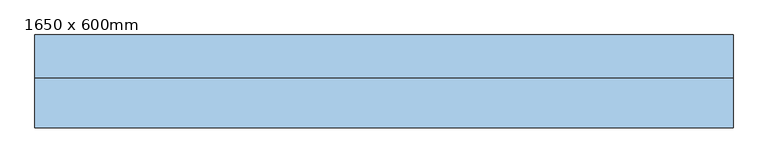
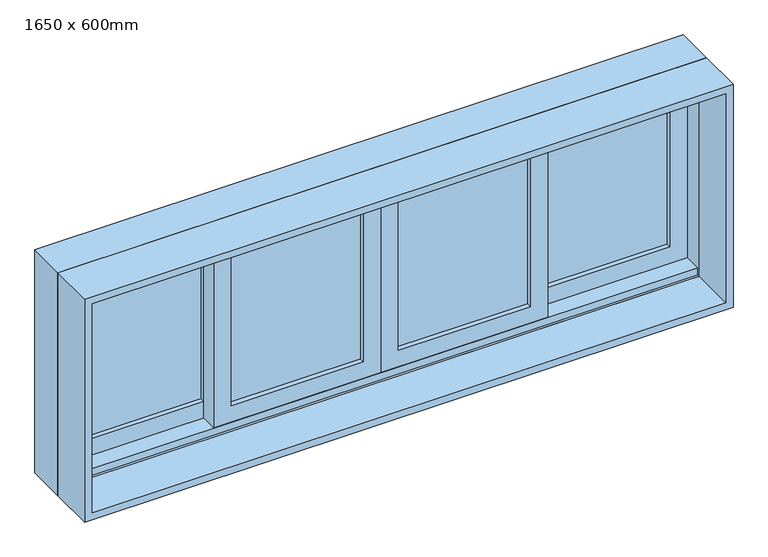
"""IFC4 building model written with IfcOpenShell, lengths in millimetres: window geometry, Janela-deslizante-quatro : 1650 x 600mm."""

import ifcopenshell
import ifcopenshell.guid

model = None  # the IFC model being written
_history = None  # IfcOwnerHistory: only IFC2X3 demands one
_inside = {}  # id of a spatial element -> (the spatial element, [elements in it])
_under = {}  # id of a project, library or spatial element -> (it, [spatial elements below it])
_declared = {}  # id of a project -> (the project, [libraries it declares])
_typed = {}  # id of a type object -> (the type object, [elements of that type])
_made_of = {}  # id of a material, layer set ... -> (it, [elements and type objects made of it])


def new_model(schema):
    """Start an empty IFC model of exactly this schema.

    Asked for "IFC4X3", IfcOpenShell would pick the latest addendum, in which some entities
    have other attributes; the version numbers below select the first issue.
    IFC2X3 requires an IfcOwnerHistory on every rooted entity: one is made here for all.
    """
    global model, _history
    if schema == "IFC4X3":
        model = ifcopenshell.file(schema_version=(4, 3, 0, 0))
    else:
        model = ifcopenshell.file(schema=schema)
    _inside.clear()
    _under.clear()
    _declared.clear()
    _typed.clear()
    _made_of.clear()
    _history = None
    if model.schema == "IFC2X3":
        org = make("IfcOrganization", Name="unknown")
        user = make(
            "IfcPersonAndOrganization",
            ThePerson=make("IfcPerson", FamilyName="unknown"),
            TheOrganization=org,
        )
        app = make(
            "IfcApplication",
            ApplicationDeveloper=org,
            Version="unknown",
            ApplicationFullName="unknown",
            ApplicationIdentifier="unknown",
        )
        _history = make(
            "IfcOwnerHistory",
            OwningUser=user,
            OwningApplication=app,
            ChangeAction="ADDED",
            CreationDate=0,
        )
    return model


def make(cls, **values):
    """One entity of the class cls with the attributes given. An attribute that is None is left unset."""
    return model.create_entity(
        cls, **{name: value for name, value in values.items() if value is not None}
    )


def rooted(cls, **values):
    """An entity with a GlobalId (a new one), such as an element, a storey or a relation."""
    return make(cls, GlobalId=ifcopenshell.guid.new(), OwnerHistory=_history, **values)


def si_unit(unit_type, name, prefix=None):
    """IfcSIUnit, for example si_unit("LENGTHUNIT", "METRE", prefix="MILLI")."""
    return make("IfcSIUnit", UnitType=unit_type, Prefix=prefix, Name=name)


def assignment(units):
    """IfcUnitAssignment: the units of a project."""
    return None if units is None else make("IfcUnitAssignment", Units=units)


def point(xyz):
    """IfcCartesianPoint."""
    return None if xyz is None else make("IfcCartesianPoint", Coordinates=xyz)


def direction(xyz):
    """IfcDirection."""
    return None if xyz is None else make("IfcDirection", DirectionRatios=xyz)


def frame(location, z_axis=None, x_axis=None):
    """IfcAxis2Placement3D, a coordinate frame: its origin and axes. An axis left out is left unset."""
    return make(
        "IfcAxis2Placement3D",
        Location=point(location),
        Axis=direction(z_axis),
        RefDirection=direction(x_axis),
    )


def origin():
    """The frame at (0, 0, 0) with its axes left unset."""
    return frame((0.0, 0.0, 0.0))


def place(relative_to, where):
    """IfcLocalPlacement: puts the frame where relative to a parent placement (None: the world)."""
    return make(
        "IfcLocalPlacement", PlacementRelTo=relative_to, RelativePlacement=where
    )


def context(
    kind, dimensions, precision=None, world=None, true_north=None, identifier=None
):
    """IfcGeometricRepresentationContext, for example the 3D "Model" context."""
    return make(
        "IfcGeometricRepresentationContext",
        ContextIdentifier=identifier,
        ContextType=kind,
        CoordinateSpaceDimension=dimensions,
        Precision=precision,
        WorldCoordinateSystem=world,
        TrueNorth=true_north,
    )


def project(units=None, contexts=None):
    """IfcProject with its units and contexts."""
    return rooted(
        "IfcProject",
        Name="project",
        RepresentationContexts=contexts,
        UnitsInContext=assignment(units),
    )


def spatial(cls, under=None, at=None, **own):
    """A site, building, storey or space (cls), placed at a placement, below another one or the project."""
    s = rooted(cls, ObjectPlacement=at, **own)
    if under is not None:
        _under.setdefault(under.id(), (under, []))[1].append(s)
    return s


def polyline(points):
    """IfcPolyline through the points."""
    return make("IfcPolyline", Points=[point(p) for p in points])


def outline(outer, holes=None, kind="AREA"):
    """IfcArbitraryClosedProfileDef: a profile drawn as a closed curve; with holes, ...WithVoids."""
    if holes is None:
        return make("IfcArbitraryClosedProfileDef", ProfileType=kind, OuterCurve=outer)
    return make(
        "IfcArbitraryProfileDefWithVoids",
        ProfileType=kind,
        OuterCurve=outer,
        InnerCurves=holes,
    )


def extrude(swept, where, along, depth):
    """IfcExtrudedAreaSolid: the profile swept, set in the frame where, extruded along a direction by depth."""
    return make(
        "IfcExtrudedAreaSolid",
        SweptArea=swept,
        Position=where,
        ExtrudedDirection=direction(along),
        Depth=depth,
    )


def faces_of(points, faces, orient=None, outer=None):
    """IfcFace entities. A face is a list of loops; a loop is a list of indices into points, from 0.

    orient and outer hold one flag for each loop. By default every Orientation is true, the
    first loop of a face is its IfcFaceOuterBound and the others are IfcFaceBound.
    """
    made = []
    for i, loops in enumerate(faces):
        bounds = []
        for j, loop in enumerate(loops):
            is_outer = j == 0 if outer is None else outer[i][j]
            bounds.append(
                make(
                    "IfcFaceOuterBound" if is_outer else "IfcFaceBound",
                    Bound=make("IfcPolyLoop", Polygon=[points[k] for k in loop]),
                    Orientation=True if orient is None else orient[i][j],
                )
            )
        made.append(make("IfcFace", Bounds=bounds))
    return made


def faceted_brep(points, faces, orient=None, outer=None, voids=None):
    """IfcFacetedBrep: a solid bounded by flat faces; with voids (closed shells), ...WithVoids."""
    shared = [point(p) for p in points]
    hull = make("IfcClosedShell", CfsFaces=faces_of(shared, faces, orient, outer))
    if voids is None:
        return make("IfcFacetedBrep", Outer=hull)
    return make(
        "IfcFacetedBrepWithVoids",
        Outer=hull,
        Voids=[
            make(cls, CfsFaces=faces_of(shared, fs, o, b)) for cls, fs, o, b in voids
        ],
    )


def shape(context_of_items, identifier, shape_type, items):
    """IfcShapeRepresentation: the items that make up one representation, for example the "Body"."""
    return make(
        "IfcShapeRepresentation",
        ContextOfItems=context_of_items,
        RepresentationIdentifier=identifier,
        RepresentationType=shape_type,
        Items=items,
    )


def source(mapping_origin, context_of_items, identifier, shape_type, items):
    """IfcRepresentationMap: a shape defined once, which mapped items show again and again."""
    return make(
        "IfcRepresentationMap",
        MappingOrigin=mapping_origin,
        MappedRepresentation=shape(context_of_items, identifier, shape_type, items),
    )


def transform(
    local_origin,
    x_axis=None,
    y_axis=None,
    z_axis=None,
    scale=None,
    scale2=None,
    scale3=None,
    uniform=True,
):
    """IfcCartesianTransformationOperator3D, or its non-uniform kind. x_axis, y_axis, z_axis: its Axis1, 2, 3."""
    if uniform:
        return make(
            "IfcCartesianTransformationOperator3D",
            Axis1=direction(x_axis),
            Axis2=direction(y_axis),
            LocalOrigin=point(local_origin),
            Scale=scale,
            Axis3=direction(z_axis),
        )
    return make(
        "IfcCartesianTransformationOperator3DnonUniform",
        Axis1=direction(x_axis),
        Axis2=direction(y_axis),
        LocalOrigin=point(local_origin),
        Scale=scale,
        Axis3=direction(z_axis),
        Scale2=scale2,
        Scale3=scale3,
    )


def mapped(mapping_source, mapping_target):
    """IfcMappedItem: shows the shape of a source again, moved by a transform."""
    return make(
        "IfcMappedItem", MappingSource=mapping_source, MappingTarget=mapping_target
    )


def made_of(thing, what):
    """Note that an element or type object is made of a material, layer set ...; save() writes the relation."""
    if what is not None:
        _made_of.setdefault(what.id(), (what, []))[1].append(thing)
    return thing


def element(
    cls,
    number,
    at=None,
    inside=None,
    cuts=None,
    type_object=None,
    material=None,
    context=None,
    identifier="Body",
    shape_type=None,
    held_by="IfcProductDefinitionShape",
    body=None,
    shapes=None,
    **own,
):
    """One element of the class cls, such as IfcWall. Its Tag is "e" and its number.

    at: its placement. inside: the storey or other place that contains it. cuts: it is an
    opening in that element (IfcRelVoidsElement). A single representation is given by context,
    identifier, shape_type and body (its items); several are given by shapes. held_by: the class
    of the entity that holds the representations. save() writes the other relations.
    """
    e = rooted(cls, Tag="e%d" % number, ObjectPlacement=at, **own)
    if body is not None:
        shapes = [shape(context, identifier, shape_type, body)]
    if shapes is not None:
        e.Representation = make(held_by, Representations=shapes)
    if inside is not None:
        _inside.setdefault(inside.id(), (inside, []))[1].append(e)
    if cuts is not None:
        rooted(
            "IfcRelVoidsElement", RelatingBuildingElement=cuts, RelatedOpeningElement=e
        )
    if type_object is not None:
        _typed.setdefault(type_object.id(), (type_object, []))[1].append(e)
    return made_of(e, material)


def aggregate(whole, parts):
    """IfcRelAggregates: a whole, such as a stair, and the parts it consists of."""
    return rooted("IfcRelAggregates", RelatingObject=whole, RelatedObjects=parts)


def save(model, path):
    """Write the relations noted so far, then the file.

    IfcRelAggregates (storeys below a building ...), IfcRelContainedInSpatialStructure (elements
    in a storey), IfcRelDefinesByType, IfcRelAssociatesMaterial and IfcRelDeclares: one each for
    every whole, place, type object, material and project.
    """
    for whole, parts in _under.values():
        aggregate(whole, parts)
    for where, things in _inside.values():
        rooted(
            "IfcRelContainedInSpatialStructure",
            RelatedElements=things,
            RelatingStructure=where,
        )
    for kind, things in _typed.values():
        rooted("IfcRelDefinesByType", RelatedObjects=things, RelatingType=kind)
    for what, things in _made_of.values():
        rooted("IfcRelAssociatesMaterial", RelatedObjects=things, RelatingMaterial=what)
    for by, libraries in _declared.values():
        rooted("IfcRelDeclares", RelatingContext=by, RelatedDefinitions=libraries)
    model.write(path)


def window_1650_x_600mm_cc7a0208(model_context):
    return source(origin(), model_context, "Body", "SolidModel", [
        faceted_brep([(-825.0, 13.64, 900.0), (-825.0, 115.24, 900.0), (825.0, 115.24, 900.0), (825.0, 13.64, 900.0), (-784.0778905, 115.24, 1459.0778905), (-784.0778905, 108.89, 1459.0778905), (-784.0778905, 108.89, 919.05), (-784.0778905, 115.24, 919.05), (784.0778905, 108.89, 1459.0778905), (784.0778905, 108.89, 919.05), (805.95, 108.89, 919.05), (805.95, 108.89, 1480.95), (-805.95, 108.89, 1480.95), (-805.95, 108.89, 919.05), (-805.95, 13.64, 1480.95), (-805.95, 13.64, 919.05), (-805.95, 19.99, 919.05), (-805.95, 19.99, 938.1), (-805.95, 64.44, 938.1), (-805.95, 64.44, 919.05), (825.0, 13.64, 1500.0), (-825.0, 13.64, 1500.0), (805.95, 13.64, 1480.95), (805.95, 13.64, 919.05), (-825.0, 115.24, 1500.0), (825.0, 115.24, 1500.0), (784.0778905, 115.24, 919.05), (784.0778905, 115.24, 1459.0778905), (805.95, 64.44, 919.05), (805.95, 64.44, 938.1), (805.95, 19.99, 938.1), (805.95, 19.99, 919.05)], [[[0, 1, 2, 3]], [[4, 5, 6, 7]], [[5, 8, 9, 10, 11, 12, 13, 6]], [[12, 14, 15, 16, 17, 18, 19, 13]], [[0, 3, 20, 21], [22, 23, 15, 14]], [[24, 1, 0, 21]], [[2, 1, 24, 25], [4, 7, 26, 27]], [[5, 4, 27, 8]], [[12, 11, 22, 14]], [[21, 20, 25, 24]], [[8, 27, 26, 9]], [[22, 11, 10, 28, 29, 30, 31, 23]], [[20, 3, 2, 25]], [[26, 7, 6, 13, 19, 28, 10, 9]], [[28, 19, 18, 29]], [[29, 18, 17, 30]], [[30, 17, 16, 31]], [[15, 23, 31, 16]]]),
        extrude(outline(polyline([(919.05, 805.95), (1480.95, 805.95), (1480.95, 380.75), (919.05, 380.75), (919.05, 805.95)]), holes=[polyline([(1436.5, 425.2), (1436.5, 761.5), (982.55, 761.5), (982.55, 425.2), (1436.5, 425.2)])]), frame((0.0, 64.44, 0.0), z_axis=(0.0, 1.0, 0.0), x_axis=(0.0, 0.0, 1.0)), (0.0, 0.0, 1.0), 44.45),
        extrude(outline(polyline([(761.5, 96.19), (761.5, 89.84), (425.2, 89.84), (425.2, 96.19), (761.5, 96.19)])), frame((0.0, 0.0, 982.55), z_axis=(0.0, 0.0, 1.0), x_axis=(1.0, 0.0, 0.0)), (0.0, 0.0, 1.0), 453.95),
        extrude(outline(polyline([(761.5, 83.1725303), (761.5, 77.14), (425.2, 77.14), (425.2, 83.1725303), (761.5, 83.1725303)])), frame((0.0, 0.0, 982.55), z_axis=(0.0, 0.0, 1.0), x_axis=(1.0, 0.0, 0.0)), (0.0, 0.0, 1.0), 453.95),
        extrude(outline(polyline([(380.75, 51.74), (380.75, 45.39), (44.45, 45.39), (44.45, 51.74), (380.75, 51.74)])), frame((0.0, 0.0, 982.55), z_axis=(0.0, 0.0, 1.0), x_axis=(1.0, 0.0, 0.0)), (0.0, 0.0, 1.0), 453.95),
        extrude(outline(polyline([(380.75, 39.04), (380.75, 32.69), (44.45, 32.69), (44.45, 39.04), (380.75, 39.04)])), frame((0.0, 0.0, 982.55), z_axis=(0.0, 0.0, 1.0), x_axis=(1.0, 0.0, 0.0)), (0.0, 0.0, 1.0), 453.95),
        extrude(outline(polyline([(1480.95, -425.2), (938.1, -425.2), (938.1, 0.0), (1480.95, 0.0), (1480.95, -425.2)]), holes=[polyline([(1436.5, -44.45), (982.55, -44.45), (982.55, -380.75), (1436.5, -380.75), (1436.5, -44.45)])]), frame((0.0, 19.99, 0.0), z_axis=(0.0, 1.0, 0.0), x_axis=(0.0, 0.0, 1.0)), (0.0, 0.0, 1.0), 44.45),
        extrude(outline(polyline([(938.1, 425.2), (1480.95, 425.2), (1480.95, 0.0), (938.1, 0.0), (938.1, 425.2)]), holes=[polyline([(982.55, 44.45), (1436.5, 44.45), (1436.5, 380.75), (982.55, 380.75), (982.55, 44.45)])]), frame((0.0, 19.99, 0.0), z_axis=(0.0, 1.0, 0.0), x_axis=(0.0, 0.0, 1.0)), (0.0, 0.0, 1.0), 44.45),
        extrude(outline(polyline([(1500.0, -825.0), (900.0, -825.0), (900.0, 825.0), (1500.0, 825.0), (1500.0, -825.0)]), holes=[polyline([(1480.95, 805.95), (919.05, 805.95), (919.05, -805.95), (1480.95, -805.95), (1480.95, 805.95)])]), frame((0.0, -103.81, 0.0), z_axis=(0.0, 1.0, 0.0), x_axis=(0.0, 0.0, 1.0)), (0.0, 0.0, 1.0), 117.45),
        extrude(outline(polyline([(-44.45, 51.74), (-44.45, 45.39), (-380.75, 45.39), (-380.75, 51.74), (-44.45, 51.74)])), frame((0.0, 0.0, 982.55), z_axis=(0.0, 0.0, 1.0), x_axis=(1.0, 0.0, 0.0)), (0.0, 0.0, 1.0), 453.95),
        extrude(outline(polyline([(-44.45, 39.04), (-44.45, 32.69), (-380.75, 32.69), (-380.75, 39.04), (-44.45, 39.04)])), frame((0.0, 0.0, 982.55), z_axis=(0.0, 0.0, 1.0), x_axis=(1.0, 0.0, 0.0)), (0.0, 0.0, 1.0), 453.95),
        extrude(outline(polyline([(-425.2, 96.19), (-425.2, 89.84), (-761.5, 89.84), (-761.5, 96.19), (-425.2, 96.19)])), frame((0.0, 0.0, 982.55), z_axis=(0.0, 0.0, 1.0), x_axis=(1.0, 0.0, 0.0)), (0.0, 0.0, 1.0), 453.95),
        extrude(outline(polyline([(-425.2, 83.49), (-425.2, 77.14), (-761.5, 77.14), (-761.5, 83.49), (-425.2, 83.49)])), frame((0.0, 0.0, 982.55), z_axis=(0.0, 0.0, 1.0), x_axis=(1.0, 0.0, 0.0)), (0.0, 0.0, 1.0), 453.95),
        extrude(outline(polyline([(919.05, -805.95), (919.05, -380.75), (1480.95, -380.75), (1480.95, -805.95), (919.05, -805.95)]), holes=[polyline([(1436.5, -425.2), (982.55, -425.2), (982.55, -761.5), (1436.5, -761.5), (1436.5, -425.2)])]), frame((0.0, 64.44, 0.0), z_axis=(0.0, 1.0, 0.0), x_axis=(0.0, 0.0, 1.0)), (0.0, 0.0, 1.0), 44.45),
    ])


if __name__ == "__main__":
    model = new_model("IFC4")
    model_context = context("Model", 3, world=origin())
    ifc_project = project(units=[si_unit("LENGTHUNIT", "METRE", prefix="MILLI")], contexts=[model_context])
    site = spatial("IfcSite", under=ifc_project)
    building = spatial("IfcBuilding", under=site)
    placement = place(None, origin())
    window_1650_x_600mm_shape = window_1650_x_600mm_cc7a0208(model_context)
    element("IfcWindow", 1, ObjectType="Janela-deslizante-quatro : 1650 x 600mm", at=placement, inside=building, context=model_context, shape_type="MappedRepresentation", body=[
        mapped(window_1650_x_600mm_shape, transform((0.0, 0.0, 0.0), x_axis=(1.0, 0.0, 0.0), y_axis=(0.0, 1.0, 0.0), z_axis=(0.0, 0.0, 1.0))),
    ])
    save(model, "model.ifc")

# Revit data of these elements
# Type "Janela-deslizante-quatro : 1650 x 600mm"
#   Type Mark = "37"
#   Classificação de incêndio = "0.5h"
#   Assembly Code = "B2020100"
#   Analytic Construction = "Vidraça dupla – residencial"
#   Janela aplicada [instance default] = 0.000 m
#   Espessura da parede [instance default] = 0.150 m
#   Visual Light Transmittance = 0.81
#   Thermal Resistance (R) = 0.319569 (m²·K)/W
#   Solar Heat Gain Coefficient = 0.76
#   Fechamento da parede interior [instance default] = 0.06745 m
#   Heat Transfer Coefficient (U) = 3.12929 W/(m²·K)
#   Extensão do quadro [instance default] = 0.00635 m
#   Fechamento da parede externa [instance default] = 0.03175 m
#   Rough Width = 1.665 m
#   Rough Height = 0.615 m
#   Height = 0.600 m
#   Umbral da extensão [instance default] = 0.06745 m
#   Altura-padrão do peitoril = 0.900 m
#   Width = 1.650 m
#   Visibilidade do montante central = yes
#   Visibilidade do recorte interior [instance default] = yes
#   Visibilidade do indicador [instance default] = yes
#   Visibilidade da apara externa [instance default] = yes
#   Visibilidade do montante lateral = yes
#   Visibilidade do umbral da extensão [instance default] = yes
#   Material da apara interior = Madeira – Manchada
#   Padrão do montante = M_Padrão do montante_2x2 : M_Padrão do montante_2x2
#   Recorte interior = M_Moldura-janela-interior-plana : Quadro
#   Material da moldura interior = Madeira – Manchada
#   Material do painel de vidro = Vidro
#   Material da apara externa = Revestimento – Branco
#   Apara externa = M_Recorte-Janela-Exterior-Plana : com peitoril
#   Material da moldura exterior = Revestimento – Branco
#   Wall Closure = (empty or 0)
# Element 1 (IfcWindow, "Janela-deslizante-quatro : 1650 x 600mm")
#   Espessura da parede = 0.200 m
#   Umbral da extensão = 0.11745 m
#   Materials on its faces: "Madeira – Manchada", "Vidro", "Revestimento – Branco"
# Materials
#   "Madeira – Manchada": class "Madeira", colour RGB 224 178 126, transparency 0, Cost = 0
#   "Vidro": class "Vidro", colour RGB 0 128 192, transparency 0.9, Description = "Vidro de sílica", Cost = 0
#   "Revestimento – Branco": class "Madeira", colour RGB 242 242 238, transparency 0, Cost = 0
